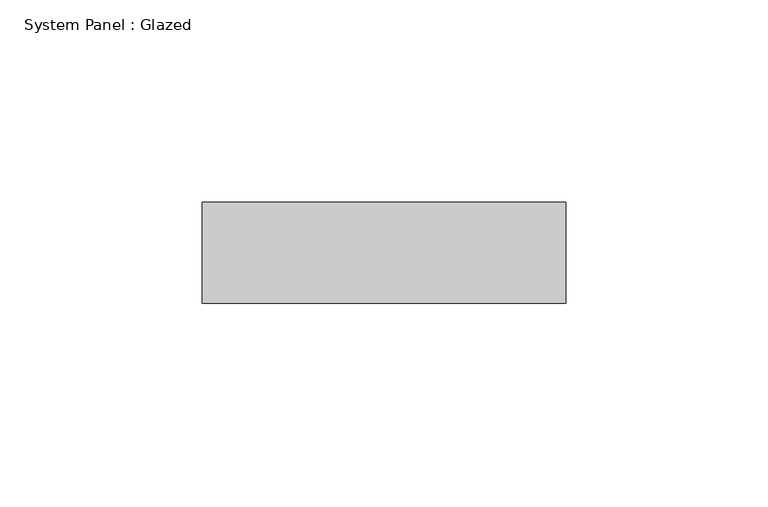
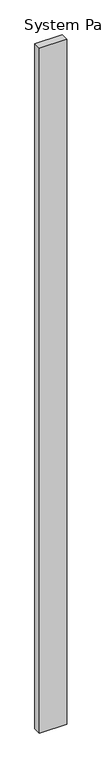
"""IFC4 building model written with IfcOpenShell, lengths in millimetres: plate geometry, System Panel : Glazed."""

from ifc_helpers import new_model, si_unit, origin, origin_with_axes, place, context, project, spatial, polyline, outline, extrude, source, transform, mapped, element, save


def system_panel_glazed_fee37a4f(model_context):
    return source(origin(), model_context, "Body", "SweptSolid", [
        extrude(outline(polyline([(44.9999998, 24.5), (-44.9999998, 24.5), (-44.9999998, 49.5), (44.9999998, 49.5), (44.9999998, 24.5)])), origin_with_axes(), (0.0, 0.0, 1.0), 2375.0),
    ])


if __name__ == "__main__":
    model = new_model("IFC4")
    model_context = context("Model", 3, world=origin())
    ifc_project = project(units=[si_unit("LENGTHUNIT", "METRE", prefix="MILLI")], contexts=[model_context])
    site = spatial("IfcSite", under=ifc_project)
    building = spatial("IfcBuilding", under=site)
    placement = place(None, origin())
    system_panel_glazed_shape = system_panel_glazed_fee37a4f(model_context)
    element("IfcPlate", 1, ObjectType="System Panel : Glazed", at=placement, inside=building, context=model_context, shape_type="MappedRepresentation", body=[
        mapped(system_panel_glazed_shape, transform((0.0, 0.0, 0.0), x_axis=(1.0, 0.0, 0.0), y_axis=(0.0, 1.0, 0.0), z_axis=(0.0, 0.0, 1.0))),
    ])
    save(model, "model.ifc")

# Revit data of these elements
# Element 1 (IfcPlate, "System Panel : Glazed")
#   Materials on its faces: "Glass"
# Materials
#   "Glass": class "Glass", colour RGB 218 227 224, transparency 0.85, Description = "Soda Lime Glass", Cost = 0
